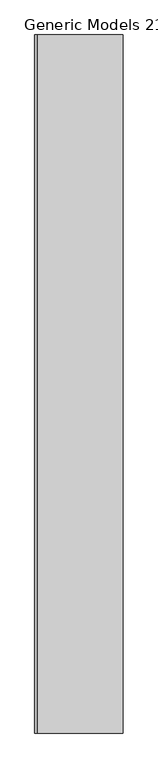
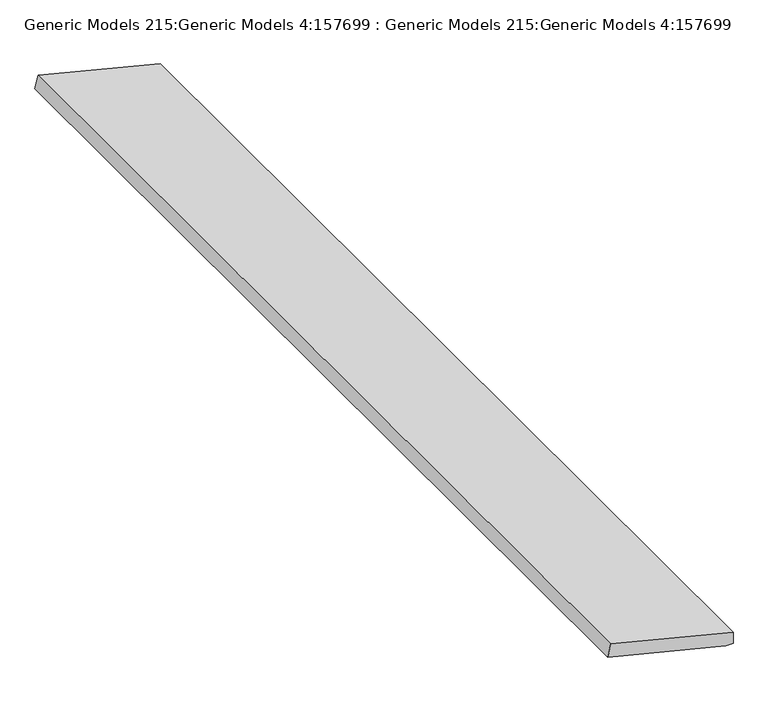
"""IFC4 building model written with IfcOpenShell, lengths in millimetres: proxy geometry, Generic Models 215:Generic Models 4:157699 : Generic Models 215:Generic Models 4:157699."""

from ifc_helpers import new_model, si_unit, frame, origin, place, context, project, spatial, polyline, outline, extrude, source, transform, mapped, element, save


def generic_models_215_generic_models_4_157699_generic_models_ff4495e3(model_context):
    return source(origin(), model_context, "Body", "SweptSolid", [
        extrude(outline(polyline([(6218.1368229, 1577.853213), (6438.4836, 1577.853213), (7012.8290519, -719.5285948), (6772.5732618, -779.5925423), (6218.1368229, 1438.153213), (6218.1368229, 1577.853213)])), frame((0.0, -6674.7974793, 0.0), z_axis=(0.0, 1.0, 0.0), x_axis=(0.0, 0.0, 1.0)), (0.0, 0.0, 1.0), 18643.6),
    ])


if __name__ == "__main__":
    model = new_model("IFC4")
    model_context = context("Model", 3, world=origin())
    ifc_project = project(units=[si_unit("LENGTHUNIT", "METRE", prefix="MILLI")], contexts=[model_context])
    site = spatial("IfcSite", under=ifc_project)
    building = spatial("IfcBuilding", under=site)
    placement = place(None, origin())
    generic_models_215_generic_models_4_157699_generic_models_shape = generic_models_215_generic_models_4_157699_generic_models_ff4495e3(model_context)
    element("IfcBuildingElementProxy", 1, Name="Generic Models 215:Generic Models 4:157699 : Generic Models 215:Generic Models 4:157699", ObjectType="Generic Models 215:Generic Models 4:157699 : Generic Models 215:Generic Models 4:157699", at=placement, inside=building, context=model_context, shape_type="MappedRepresentation", body=[
        mapped(generic_models_215_generic_models_4_157699_generic_models_shape, transform((0.0, 0.0, 0.0), x_axis=(1.0, 0.0, 0.0), y_axis=(0.0, 1.0, 0.0), z_axis=(0.0, 0.0, 1.0))),
    ])
    save(model, "model.ifc")

# Revit data of these elements
# Type "Generic Models 215:Generic Models 4:157699 : Generic Models 215:Generic Models 4:157699"
#   NameOverride = "Generic Models 215:Generic Models 4:157699"
#   ObjectTypeOverride = "Generic Models 215:Generic Models 4"
#   Reference = "Generic Models 4"
#   Category = "Generic Models"
#   Tag = "157699"
# Element 1 (IfcBuildingElementProxy, "Generic Models 215:Generic Models 4:157699 : Generic Models 215:Generic Models 4:157699")
#   Materials on its faces: "_BATT INSUL. (R-FACTOR = R30 MIN) OVER CLASS II VAPOR RETARDER(TOWARD INTERIOR) 50493"
# Materials
#   "_BATT INSUL. (R-FACTOR = R30 MIN) OVER CLASS II VAPOR RETARDER(TOWARD INTERIOR) 50493": class "Unassigned", colour RGB 200 166 247, transparency 0
